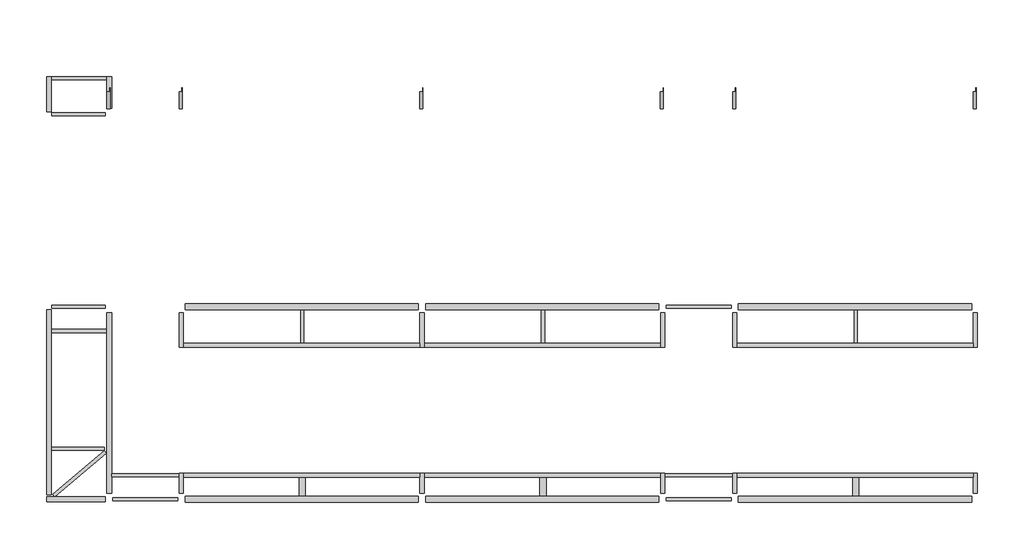
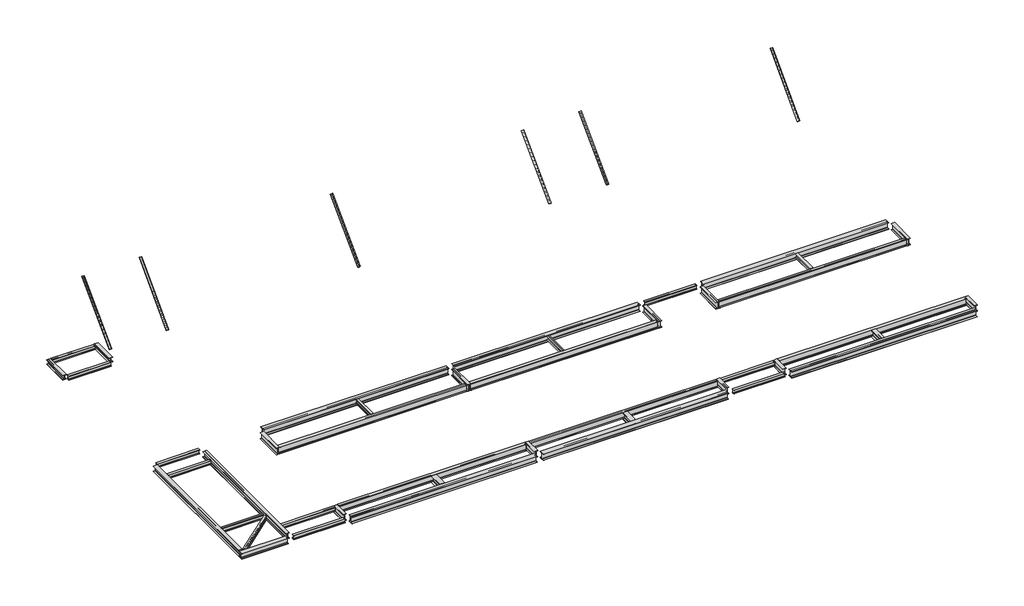
# One storey: 50 beams.
# Revit data of these elements (continued)
# Project information (continued)
#   H_Project Abbreviation = "SACE"
#   Project Status = "Project Status"
#   Client Name = "현대엔지니어링"
#   Project Address = "서울시 종로구 율곡로 75(계동)"
#   Project Name = "Jafurah"
#   Project Number = "-"
# Grids (mm)
#   "25": line (-6469.284, 5499.521) -> (39003.298, 5499.521)
#   "26": line (-1950, 24502.793) -> (-1950, -3987.031)
#   "27": line (37500, 24502.793) -> (37500, -3987.031)
#   "30": line (-6469.284, 7499.521) -> (39003.298, 7499.521)
#   "34": line (-6469.284, 13499.521) -> (39003.298, 13499.521)
#   "35": line (-6469.284, 15499.521) -> (39003.298, 15499.521)
#   "37": line (-6469.284, 21499.521) -> (39003.298, 21499.521)
#   "40": line (-6469.284, -500.479) -> (39003.298, -500.479)
#   "41": line (-6469.284, 1499.521) -> (39003.298, 1499.521)
#   "D": line (-6469.284, 22499.521) -> (39003.298, 22499.521)
#   "1": line (0, 24502.793) -> (0, -3987.031)
#   "3": line (13000, 24502.793) -> (13000, -3987.031)
#   "B": line (-6469.284, 6499.521) -> (39003.298, 6499.521)
#   "A": line (-6469.284, 499.521) -> (39003.298, 499.521)
#   "4": line (23000, 24502.793) -> (23000, -3987.031)
#   "5": line (26000, 24502.793) -> (26000, -3987.031)
#   "6": line (36000, 24502.793) -> (36000, -3987.031)
#   "1 A": line (-2500, 24502.793) -> (-2500, 12276.643)
#   "2": line (3000, 24502.793) -> (3000, -3987.031)
#   "7": line (1307.038, 15699.521) -> (-4718.233, 15699.521)
#   "8": line (1307.038, 17449.521) -> (-4718.233, 17449.521)
#   "9": line (5528.605, 13006.092) -> (5528.605, 16811.527)
#   "10": line (8028.605, 13006.092) -> (8028.605, 16811.527)
#   "11": line (10528.605, 13006.092) -> (10528.605, 16811.527)
#   "12": line (20528.605, 13006.092) -> (20528.605, 16811.527)
#   "13": line (18028.605, 13006.092) -> (18028.605, 16811.527)
#   "14": line (15528.605, 13006.092) -> (15528.605, 16811.527)
#   "15": line (18000, -1079.942) -> (18000, 22499.521)
#   "16": line (27211.823, 9169.521) -> (22203.608, 9169.521)
#   "17": line (3430.624, 9199.521) -> (-461.103, 9199.521)
#   "18": line (4961.493, 9299.521) -> (2471.526, 9299.521)
#   "19": line (20500, 22120.772) -> (20500, 25499.521)
#   "20": line (15500, 22120.772) -> (15500, 25499.521)
#   "21": line (10500, 22120.772) -> (10500, 25499.521)
#   "22": line (5500, 22120.772) -> (5500, 25499.521)
#   "23": line (-6469.284, -2000.479) -> (39003.298, -2000.479)
#   "C": line (-6469.284, 14499.521) -> (39003.298, 14499.521)
# Type "0912_Steel Framing_L-KSD3502 : H_SB_AR_S04_L-130x130x12_KBR1"
#   k = 25 mm
#   Perimeter = 0.52 m²/m
#   Nominal Weight = 23.40 kgf/m
#   Length [instance default] = 1000 mm
#   b = 130 mm
#   d = 130 mm
#   t = 12 mm
#   x = 36.4 mm
#   y = 36.4 mm
#   A = 2976.00 m²
#   Structural Material [instance default] = Steel, 45-345
# Type "Steel Framing_W_ASTM A6M : H_SB_AR_S02_W200x31.3_B6"
#   Type Mark = "B6"
#   Section Name Key = "W8x21"
#   Width = 13.4 cm
#   Web Thickness = 0.635 cm
#   Web Fillet = 0.76 cm
#   Warping Constant = 40800.0 cm⁶
#   Torsional Moment of Inertia = 11.70 cm⁴
#   Section Area = 39.7 cm²
#   Plastic Modulus weak axis = 93.2 cm³
#   Plastic Modulus strong axis = 334.0 cm³
#   Perimeter = 0.93 m²/m
#   Nominal Weight = 31.30 kgf/m
#   Moment of Inertia weak axis = 407.00 cm⁴
#   Moment of Inertia strong axis = 3130.00 cm⁴
#   Height = 21.0 cm
#   Flange Thickness = 1.02 cm
#   Elastic Modulus weak axis = 60.8 cm³
#   Elastic Modulus strong axis = 298.0 cm³
#   Centroid Vertical = 10.5 cm
#   Centroid Horizontal = 6.7 cm
#   Length [instance default] = 1500 mm
#   Structural Material [instance default] = Steel, 45-345
#   Bolt Spacing = 0
#   Assembly Code = ""
# Type "Steel Framing_W_ASTM A6M : H_SB_AR_S02_W360x91_B3"
#   Type Mark = "B3"
#   Section Name Key = "W14x61"
#   Width = 25.4 cm
#   Web Thickness = 0.953 cm
#   Web Fillet = 1.51 cm
#   Warping Constant = 1260000.0 cm⁶
#   Torsional Moment of Inertia = 91.20 cm⁴
#   Section Area = 115.0 cm²
#   Plastic Modulus weak axis = 537.0 cm³
#   Plastic Modulus strong axis = 1670.0 cm³
#   Perimeter = 1.68 m²/m
#   Nominal Weight = 91.00 kgf/m
#   Moment of Inertia weak axis = 4450.00 cm⁴
#   Moment of Inertia strong axis = 26600.00 cm⁴
#   Height = 35.3 cm
#   Flange Thickness = 1.64 cm
#   Elastic Modulus weak axis = 352.0 cm³
#   Elastic Modulus strong axis = 1510.0 cm³
#   Centroid Vertical = 17.65 cm
#   Centroid Horizontal = 12.7 cm
#   Length [instance default] = 1500 mm
#   Structural Material [instance default] = Steel, 45-345
#   Bolt Spacing = 0
#   Assembly Code = ""
# Type "Steel Framing_W_ASTM A6M : H_SB_AR_S02_W310x60_G4"
#   Type Mark = "G4"
#   Section Name Key = "W12x40"
#   Width = 20.3 cm
#   Web Thickness = 0.749 cm
#   Web Fillet = 1.28 cm
#   Warping Constant = 387000.0 cm⁶
#   Torsional Moment of Inertia = 37.70 cm⁴
#   Section Area = 75.5 cm²
#   Plastic Modulus weak axis = 275.0 cm³
#   Plastic Modulus strong axis = 934.0 cm³
#   Perimeter = 1.38 m²/m
#   Nominal Weight = 60.00 kgf/m
#   Moment of Inertia weak axis = 1840.00 cm⁴
#   Moment of Inertia strong axis = 12800.00 cm⁴
#   Height = 30.2 cm
#   Flange Thickness = 1.31 cm
#   Elastic Modulus weak axis = 180.0 cm³
#   Elastic Modulus strong axis = 844.0 cm³
#   Centroid Vertical = 15.1 cm
#   Centroid Horizontal = 10.15 cm
#   Length [instance default] = 1500 mm
#   Structural Material [instance default] = Steel, 45-345
#   Bolt Spacing = 0
#   Assembly Code = ""
# Type "Steel Framing_W_ASTM A6M : H_SB_AR_S02_W250x49.1_G5"
#   Type Mark = "G5"
#   Section Name Key = "W10x33"
#   Width = 20.2 cm
#   Web Thickness = 0.737 cm
#   Web Fillet = 1.27 cm
#   Warping Constant = 212000.0 cm⁶
#   Torsional Moment of Inertia = 24.30 cm⁴
#   Section Area = 62.6 cm²
#   Plastic Modulus weak axis = 229.0 cm³
#   Plastic Modulus strong axis = 636.0 cm³
#   Perimeter = 1.27 m²/m
#   Nominal Weight = 49.10 kgf/m
#   Moment of Inertia weak axis = 1520.00 cm⁴
#   Moment of Inertia strong axis = 7120.00 cm⁴
#   Height = 24.7 cm
#   Flange Thickness = 1.1 cm
#   Elastic Modulus weak axis = 151.0 cm³
#   Elastic Modulus strong axis = 574.0 cm³
#   Centroid Vertical = 12.35 cm
#   Centroid Horizontal = 10.1 cm
#   Length [instance default] = 1500 mm
#   Structural Material [instance default] = Steel, 45-345
#   Bolt Spacing = 0
#   Assembly Code = ""
# Type "Steel Framing_W_ASTM A6M : H_SB_AR_S02_W310x60_B5"
#   Type Mark = "B5"
#   Section Name Key = "W12x40"
#   Width = 20.3 cm
#   Web Thickness = 0.749 cm
#   Web Fillet = 1.28 cm
#   Warping Constant = 387000.0 cm⁶
#   Torsional Moment of Inertia = 37.70 cm⁴
#   Section Area = 75.5 cm²
#   Plastic Modulus weak axis = 275.0 cm³
#   Plastic Modulus strong axis = 934.0 cm³
#   Perimeter = 1.38 m²/m
#   Nominal Weight = 60.00 kgf/m
#   Moment of Inertia weak axis = 1840.00 cm⁴
#   Moment of Inertia strong axis = 12800.00 cm⁴
#   Height = 30.2 cm
#   Flange Thickness = 1.31 cm
#   Elastic Modulus weak axis = 180.0 cm³
#   Elastic Modulus strong axis = 844.0 cm³
#   Centroid Vertical = 15.1 cm
#   Centroid Horizontal = 10.15 cm
#   Length [instance default] = 1500 mm
#   Structural Material [instance default] = Steel, 45-345
#   Bolt Spacing = 0
#   Assembly Code = ""
# Type "Steel Framing_W_ASTM A6M : H_SB_AR_S02_W360x51_G3"
#   Type Mark = "G3"
#   Section Name Key = "W14x34"
#   Width = 17.1 cm
#   Web Thickness = 0.724 cm
#   Web Fillet = 1.01 cm
#   Warping Constant = 287000.0 cm⁶
#   Torsional Moment of Inertia = 23.70 cm⁴
#   Section Area = 64.5 cm²
#   Plastic Modulus weak axis = 174.0 cm³
#   Plastic Modulus strong axis = 895.0 cm³
#   Perimeter = 1.36 m²/m
#   Nominal Weight = 51.00 kgf/m
#   Moment of Inertia weak axis = 970.00 cm⁴
#   Moment of Inertia strong axis = 14200.00 cm⁴
#   Height = 35.6 cm
#   Flange Thickness = 1.16 cm
#   Elastic Modulus weak axis = 113.0 cm³
#   Elastic Modulus strong axis = 796.0 cm³
#   Centroid Vertical = 17.8 cm
#   Centroid Horizontal = 8.55 cm
#   Length [instance default] = 1500 mm
#   Structural Material [instance default] = Steel, 45-345
#   Bolt Spacing = 0
#   Assembly Code = ""
# Type "Steel Framing_W_ASTM A6M : H_SB_AR_S02_W360x51_B4"
#   Type Mark = "B4"
#   Section Name Key = "W14x34"
#   Width = 17.1 cm
#   Web Thickness = 0.724 cm
#   Web Fillet = 1.01 cm
#   Warping Constant = 287000.0 cm⁶
#   Torsional Moment of Inertia = 23.70 cm⁴
#   Section Area = 64.5 cm²
#   Plastic Modulus weak axis = 174.0 cm³
#   Plastic Modulus strong axis = 895.0 cm³
#   Perimeter = 1.36 m²/m
#   Nominal Weight = 51.00 kgf/m
#   Moment of Inertia weak axis = 970.00 cm⁴
#   Moment of Inertia strong axis = 14200.00 cm⁴
#   Height = 35.6 cm
#   Flange Thickness = 1.16 cm
#   Elastic Modulus weak axis = 113.0 cm³
#   Elastic Modulus strong axis = 796.0 cm³
#   Centroid Vertical = 17.8 cm
#   Centroid Horizontal = 8.55 cm
#   Length [instance default] = 1500 mm
#   Structural Material [instance default] = Steel, 45-345
#   Bolt Spacing = 0
#   Assembly Code = ""
# Elements 1, 2, 3, 4, 5, 6 (IfcBeam, "0912_Steel Framing_L-KSD3502 : H_SB_AR_S04_L-130x130x12_KBR1")
#   Structural Material = Steel ASTM A36
#   Phase Created = New Construction
#   Materials on its faces: "Steel ASTM A36"
# Elements 7, 8, 9, 10, 11, 12, 21, 23, 25, 27, 28, 45, 46, 47 (IfcBeam, "Steel Framing_W_ASTM A6M : H_SB_AR_S02_W200x31.3_B6")
#   Structural Material = Steel, 45-345
#   Phase Created = New Construction
#   Materials on its faces: "Steel, 45-345"
# Elements 13, 14, 15, 16, 17, 18, 48, 49, 50 (IfcBeam, "Steel Framing_W_ASTM A6M : H_SB_AR_S02_W360x91_B3")
#   Structural Material = Steel, 45-345
#   Phase Created = New Construction
#   Materials on its faces: "Steel, 45-345"
# Element 19 (IfcBeam, "Steel Framing_W_ASTM A6M : H_SB_AR_S02_W310x60_G4")
#   Structural Material = Steel, 45-345
#   Phase Created = New Construction
#   Materials on its faces: "Steel, 45-345"
# Elements 20, 22 (IfcBeam, "Steel Framing_W_ASTM A6M : H_SB_AR_S02_W250x49.1_G5")
#   Length = 1500 mm
#   Structural Material = Steel, 45-345
#   Phase Created = New Construction
#   Materials on its faces: "Steel, 45-345"
# Elements 24, 26 (IfcBeam, "Steel Framing_W_ASTM A6M : H_SB_AR_S02_W310x60_B5")
#   Structural Material = Steel, 45-345
#   Phase Created = New Construction
#   Materials on its faces: "Steel, 45-345"
# Elements 29, 30, 31, 32, 33, 40, 41, 42, 43, 44 (IfcBeam, "Steel Framing_W_ASTM A6M : H_SB_AR_S02_W360x51_G3")
#   Structural Material = Steel, 45-345
#   Phase Created = New Construction
#   Materials on its faces: "Steel, 45-345"
# Elements 34, 35, 36, 37, 38, 39 (IfcBeam, "Steel Framing_W_ASTM A6M : H_SB_AR_S02_W360x51_B4")
#   Structural Material = Steel, 45-345
#   Phase Created = New Construction
#   Materials on its faces: "Steel, 45-345"
# Materials
#   "Steel, 45-345": class "Metal", colour RGB 189 187 185, transparency 0, Description = "Steel 345 MPa", Cost = 0
#   "Steel ASTM A36": class "Metal", colour RGB 199 199 199, transparency 0, Description = "Structural steel, ASTM A36 Grade B, mill finish", Cost = 0
